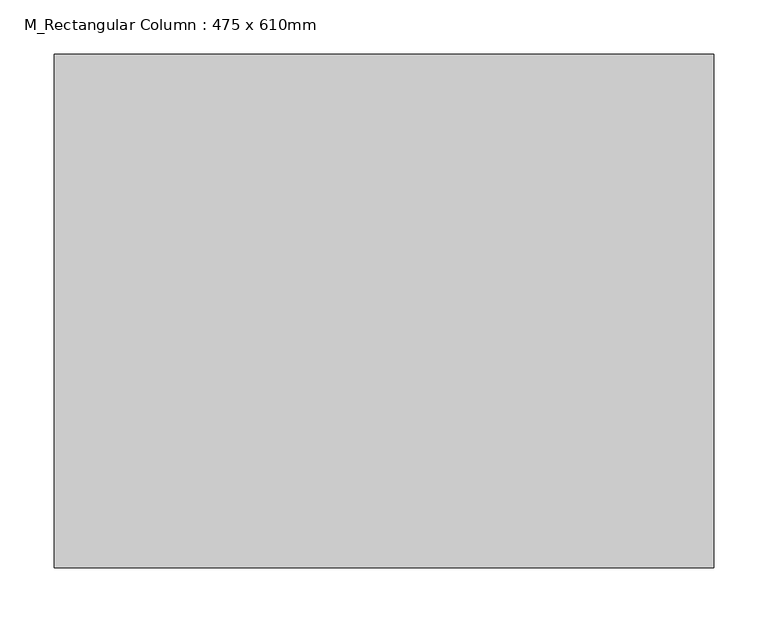
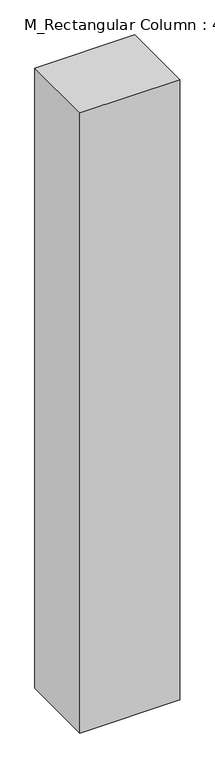
"""IFC4 building model written with IfcOpenShell, lengths in millimetres: column geometry, M_Rectangular Column : 475 x 610mm."""

import ifcopenshell
import ifcopenshell.guid

model = None  # the IFC model being written
_history = None  # IfcOwnerHistory: only IFC2X3 demands one
_inside = {}  # id of a spatial element -> (the spatial element, [elements in it])
_under = {}  # id of a project, library or spatial element -> (it, [spatial elements below it])
_declared = {}  # id of a project -> (the project, [libraries it declares])
_typed = {}  # id of a type object -> (the type object, [elements of that type])
_made_of = {}  # id of a material, layer set ... -> (it, [elements and type objects made of it])


def new_model(schema):
    """Start an empty IFC model of exactly this schema.

    Asked for "IFC4X3", IfcOpenShell would pick the latest addendum, in which some entities
    have other attributes; the version numbers below select the first issue.
    IFC2X3 requires an IfcOwnerHistory on every rooted entity: one is made here for all.
    """
    global model, _history
    if schema == "IFC4X3":
        model = ifcopenshell.file(schema_version=(4, 3, 0, 0))
    else:
        model = ifcopenshell.file(schema=schema)
    _inside.clear()
    _under.clear()
    _declared.clear()
    _typed.clear()
    _made_of.clear()
    _history = None
    if model.schema == "IFC2X3":
        org = make("IfcOrganization", Name="unknown")
        user = make(
            "IfcPersonAndOrganization",
            ThePerson=make("IfcPerson", FamilyName="unknown"),
            TheOrganization=org,
        )
        app = make(
            "IfcApplication",
            ApplicationDeveloper=org,
            Version="unknown",
            ApplicationFullName="unknown",
            ApplicationIdentifier="unknown",
        )
        _history = make(
            "IfcOwnerHistory",
            OwningUser=user,
            OwningApplication=app,
            ChangeAction="ADDED",
            CreationDate=0,
        )
    return model


def make(cls, **values):
    """One entity of the class cls with the attributes given. An attribute that is None is left unset."""
    return model.create_entity(
        cls, **{name: value for name, value in values.items() if value is not None}
    )


def rooted(cls, **values):
    """An entity with a GlobalId (a new one), such as an element, a storey or a relation."""
    return make(cls, GlobalId=ifcopenshell.guid.new(), OwnerHistory=_history, **values)


def si_unit(unit_type, name, prefix=None):
    """IfcSIUnit, for example si_unit("LENGTHUNIT", "METRE", prefix="MILLI")."""
    return make("IfcSIUnit", UnitType=unit_type, Prefix=prefix, Name=name)


def assignment(units):
    """IfcUnitAssignment: the units of a project."""
    return None if units is None else make("IfcUnitAssignment", Units=units)


def point(xyz):
    """IfcCartesianPoint."""
    return None if xyz is None else make("IfcCartesianPoint", Coordinates=xyz)


def direction(xyz):
    """IfcDirection."""
    return None if xyz is None else make("IfcDirection", DirectionRatios=xyz)


def frame(location, z_axis=None, x_axis=None):
    """IfcAxis2Placement3D, a coordinate frame: its origin and axes. An axis left out is left unset."""
    return make(
        "IfcAxis2Placement3D",
        Location=point(location),
        Axis=direction(z_axis),
        RefDirection=direction(x_axis),
    )


def origin():
    """The frame at (0, 0, 0) with its axes left unset."""
    return frame((0.0, 0.0, 0.0))


def origin_with_axes():
    """The frame at (0, 0, 0) with the z axis (0, 0, 1) and the x axis (1, 0, 0) written out."""
    return frame((0.0, 0.0, 0.0), z_axis=(0.0, 0.0, 1.0), x_axis=(1.0, 0.0, 0.0))


def place(relative_to, where):
    """IfcLocalPlacement: puts the frame where relative to a parent placement (None: the world)."""
    return make(
        "IfcLocalPlacement", PlacementRelTo=relative_to, RelativePlacement=where
    )


def context(
    kind, dimensions, precision=None, world=None, true_north=None, identifier=None
):
    """IfcGeometricRepresentationContext, for example the 3D "Model" context."""
    return make(
        "IfcGeometricRepresentationContext",
        ContextIdentifier=identifier,
        ContextType=kind,
        CoordinateSpaceDimension=dimensions,
        Precision=precision,
        WorldCoordinateSystem=world,
        TrueNorth=true_north,
    )


def project(units=None, contexts=None):
    """IfcProject with its units and contexts."""
    return rooted(
        "IfcProject",
        Name="project",
        RepresentationContexts=contexts,
        UnitsInContext=assignment(units),
    )


def spatial(cls, under=None, at=None, **own):
    """A site, building, storey or space (cls), placed at a placement, below another one or the project."""
    s = rooted(cls, ObjectPlacement=at, **own)
    if under is not None:
        _under.setdefault(under.id(), (under, []))[1].append(s)
    return s


def polyline(points):
    """IfcPolyline through the points."""
    return make("IfcPolyline", Points=[point(p) for p in points])


def outline(outer, holes=None, kind="AREA"):
    """IfcArbitraryClosedProfileDef: a profile drawn as a closed curve; with holes, ...WithVoids."""
    if holes is None:
        return make("IfcArbitraryClosedProfileDef", ProfileType=kind, OuterCurve=outer)
    return make(
        "IfcArbitraryProfileDefWithVoids",
        ProfileType=kind,
        OuterCurve=outer,
        InnerCurves=holes,
    )


def extrude(swept, where, along, depth):
    """IfcExtrudedAreaSolid: the profile swept, set in the frame where, extruded along a direction by depth."""
    return make(
        "IfcExtrudedAreaSolid",
        SweptArea=swept,
        Position=where,
        ExtrudedDirection=direction(along),
        Depth=depth,
    )


def shape(context_of_items, identifier, shape_type, items):
    """IfcShapeRepresentation: the items that make up one representation, for example the "Body"."""
    return make(
        "IfcShapeRepresentation",
        ContextOfItems=context_of_items,
        RepresentationIdentifier=identifier,
        RepresentationType=shape_type,
        Items=items,
    )


def source(mapping_origin, context_of_items, identifier, shape_type, items):
    """IfcRepresentationMap: a shape defined once, which mapped items show again and again."""
    return make(
        "IfcRepresentationMap",
        MappingOrigin=mapping_origin,
        MappedRepresentation=shape(context_of_items, identifier, shape_type, items),
    )


def transform(
    local_origin,
    x_axis=None,
    y_axis=None,
    z_axis=None,
    scale=None,
    scale2=None,
    scale3=None,
    uniform=True,
):
    """IfcCartesianTransformationOperator3D, or its non-uniform kind. x_axis, y_axis, z_axis: its Axis1, 2, 3."""
    if uniform:
        return make(
            "IfcCartesianTransformationOperator3D",
            Axis1=direction(x_axis),
            Axis2=direction(y_axis),
            LocalOrigin=point(local_origin),
            Scale=scale,
            Axis3=direction(z_axis),
        )
    return make(
        "IfcCartesianTransformationOperator3DnonUniform",
        Axis1=direction(x_axis),
        Axis2=direction(y_axis),
        LocalOrigin=point(local_origin),
        Scale=scale,
        Axis3=direction(z_axis),
        Scale2=scale2,
        Scale3=scale3,
    )


def mapped(mapping_source, mapping_target):
    """IfcMappedItem: shows the shape of a source again, moved by a transform."""
    return make(
        "IfcMappedItem", MappingSource=mapping_source, MappingTarget=mapping_target
    )


def made_of(thing, what):
    """Note that an element or type object is made of a material, layer set ...; save() writes the relation."""
    if what is not None:
        _made_of.setdefault(what.id(), (what, []))[1].append(thing)
    return thing


def element(
    cls,
    number,
    at=None,
    inside=None,
    cuts=None,
    type_object=None,
    material=None,
    context=None,
    identifier="Body",
    shape_type=None,
    held_by="IfcProductDefinitionShape",
    body=None,
    shapes=None,
    **own,
):
    """One element of the class cls, such as IfcWall. Its Tag is "e" and its number.

    at: its placement. inside: the storey or other place that contains it. cuts: it is an
    opening in that element (IfcRelVoidsElement). A single representation is given by context,
    identifier, shape_type and body (its items); several are given by shapes. held_by: the class
    of the entity that holds the representations. save() writes the other relations.
    """
    e = rooted(cls, Tag="e%d" % number, ObjectPlacement=at, **own)
    if body is not None:
        shapes = [shape(context, identifier, shape_type, body)]
    if shapes is not None:
        e.Representation = make(held_by, Representations=shapes)
    if inside is not None:
        _inside.setdefault(inside.id(), (inside, []))[1].append(e)
    if cuts is not None:
        rooted(
            "IfcRelVoidsElement", RelatingBuildingElement=cuts, RelatedOpeningElement=e
        )
    if type_object is not None:
        _typed.setdefault(type_object.id(), (type_object, []))[1].append(e)
    return made_of(e, material)


def aggregate(whole, parts):
    """IfcRelAggregates: a whole, such as a stair, and the parts it consists of."""
    return rooted("IfcRelAggregates", RelatingObject=whole, RelatedObjects=parts)


def save(model, path):
    """Write the relations noted so far, then the file.

    IfcRelAggregates (storeys below a building ...), IfcRelContainedInSpatialStructure (elements
    in a storey), IfcRelDefinesByType, IfcRelAssociatesMaterial and IfcRelDeclares: one each for
    every whole, place, type object, material and project.
    """
    for whole, parts in _under.values():
        aggregate(whole, parts)
    for where, things in _inside.values():
        rooted(
            "IfcRelContainedInSpatialStructure",
            RelatedElements=things,
            RelatingStructure=where,
        )
    for kind, things in _typed.values():
        rooted("IfcRelDefinesByType", RelatedObjects=things, RelatingType=kind)
    for what, things in _made_of.values():
        rooted("IfcRelAssociatesMaterial", RelatedObjects=things, RelatingMaterial=what)
    for by, libraries in _declared.values():
        rooted("IfcRelDeclares", RelatingContext=by, RelatedDefinitions=libraries)
    model.write(path)


def m_rectangular_column_475_x_610mm_b7c60445(model_context):
    return source(origin(), model_context, "Body", "SweptSolid", [
        extrude(outline(polyline([(305.0, 237.5), (305.0, -237.5), (-305.0, -237.5), (-305.0, 237.5), (305.0, 237.5)])), origin_with_axes(), (0.0, 0.0, 1.0), 4000.0),
    ])


if __name__ == "__main__":
    model = new_model("IFC4")
    model_context = context("Model", 3, world=origin())
    ifc_project = project(units=[si_unit("LENGTHUNIT", "METRE", prefix="MILLI")], contexts=[model_context])
    site = spatial("IfcSite", under=ifc_project)
    building = spatial("IfcBuilding", under=site)
    placement = place(None, origin())
    m_rectangular_column_475_x_610mm_shape = m_rectangular_column_475_x_610mm_b7c60445(model_context)
    element("IfcColumn", 1, ObjectType="M_Rectangular Column : 475 x 610mm", at=placement, inside=building, context=model_context, shape_type="MappedRepresentation", body=[
        mapped(m_rectangular_column_475_x_610mm_shape, transform((0.0, 0.0, 0.0), x_axis=(1.0, 0.0, 0.0), y_axis=(0.0, 1.0, 0.0), z_axis=(0.0, 0.0, 1.0))),
    ])
    save(model, "model.ifc")

# Revit data of these elements
# Project information
#   Project Issue Date = "Issue Date"
#   Project Status = "Project Status"
#   Client Name = "Owner"
#   Project Address = "Enter address here"
#   Project Name = "Project Name"
#   Project Number = "0001"
# Type "M_Rectangular Column : 475 x 610mm"
#   Depth = 475 mm
#   Offset Base = 0 mm
#   Offset Top = 0 mm
#   Width = 610 mm
#   Material = none
